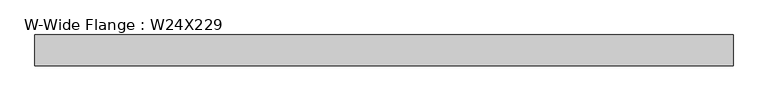
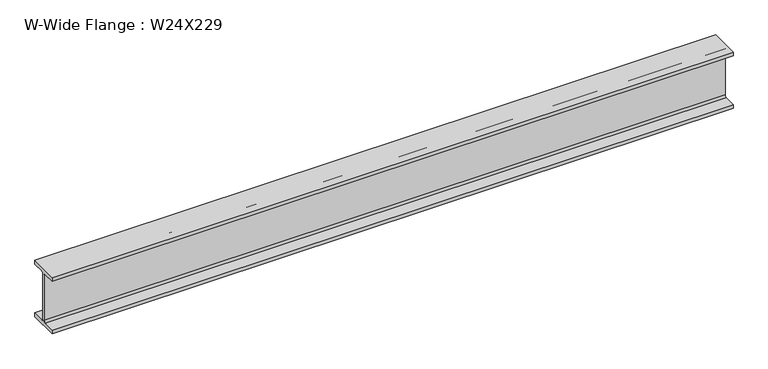
"""IFC4 building model written with IfcOpenShell, lengths in millimetres: beam geometry, W-Wide Flange : W24X229."""

from ifc_helpers import new_model, si_unit, point, frame, frame_2d, origin, place, context, project, spatial, polyline, circle_curve, trimmed, segment, composite_curve, outline, extrude, source, transform, mapped, element, save


def w_wide_flange_w24x229_eebb78a0(model_context):
    return source(origin(), model_context, "Body", "SweptSolid", [
        extrude(outline(composite_curve([segment(polyline([(-166.37, -286.258), (-34.925, -286.258)]), True, "CONTINUOUS"), segment(trimmed(circle_curve(frame_2d((-34.925, -263.525)), 22.733), [point((-34.925, -286.258))], [point((-12.192, -263.525))], True, "CARTESIAN"), True, "CONTINUOUS"), segment(polyline([(-12.192, -263.525), (-12.192, 263.525)]), True, "CONTINUOUS"), segment(trimmed(circle_curve(frame_2d((-34.925, 263.525)), 22.733), [point((-12.192, 263.525))], [point((-34.925, 286.258))], True, "CARTESIAN"), True, "CONTINUOUS"), segment(polyline([(-34.925, 286.258), (-166.37, 286.258), (-166.37, 330.2), (166.37, 330.2), (166.37, 286.258), (34.925, 286.258)]), True, "CONTINUOUS"), segment(trimmed(circle_curve(frame_2d((34.925, 263.525)), 22.733), [point((34.925, 286.258))], [point((12.192, 263.525))], True, "CARTESIAN"), True, "CONTINUOUS"), segment(polyline([(12.192, 263.525), (12.192, -263.525)]), True, "CONTINUOUS"), segment(trimmed(circle_curve(frame_2d((34.925, -263.525)), 22.733), [point((12.192, -263.525))], [point((34.925, -286.258))], True, "CARTESIAN"), True, "CONTINUOUS"), segment(polyline([(34.925, -286.258), (166.37, -286.258), (166.37, -330.2), (-166.37, -330.2), (-166.37, -286.258)]), True, "CONTINUOUS")], self_intersect=False)), frame((-3793.384977, 0.0, 0.0), z_axis=(1.0, 0.0, 0.0), x_axis=(0.0, 1.0, 0.0)), (0.0, 0.0, 1.0), 7550.785),
    ])


if __name__ == "__main__":
    model = new_model("IFC4")
    model_context = context("Model", 3, world=origin())
    ifc_project = project(units=[si_unit("LENGTHUNIT", "METRE", prefix="MILLI")], contexts=[model_context])
    site = spatial("IfcSite", under=ifc_project)
    building = spatial("IfcBuilding", under=site)
    placement = place(None, origin())
    w_wide_flange_w24x229_shape = w_wide_flange_w24x229_eebb78a0(model_context)
    element("IfcBeam", 1, ObjectType="W-Wide Flange : W24X229", at=placement, inside=building, context=model_context, shape_type="MappedRepresentation", body=[
        mapped(w_wide_flange_w24x229_shape, transform((0.0, 0.0, 0.0), x_axis=(1.0, 0.0, 0.0), y_axis=(0.0, 1.0, 0.0), z_axis=(0.0, 0.0, 1.0))),
    ])
    save(model, "model.ifc")

# Revit data of these elements
# Type "W-Wide Flange : W24X229"
#   Assembly Code = "B10"
#   W = 229
#   Start Extension Calculation [instance default] = 10' - 0"
#   Start Extension [instance default] = -0' - 0 1/2"
#   End Extension Calculation [instance default] = 10' - 0"
#   End Extension [instance default] = -0' - 0 1/2"
#   Length [instance default] = 5' - 0"
#   bf = 1' - 1.1"
#   d = 2' - 2"
#   k = 0' - 2 5/8"
#   k2 = 0' - 0.895"
#   tf = 0' - 1.73"
#   tw = 0' - 0.96"
#   A = 0.466667 SF
#   Beam Material [instance default] = Metal - Steel - ASTM A992
# Element 1 (IfcBeam, "W-Wide Flange : W24X229")
#   Materials on its faces: "Metal - Steel - ASTM A992"
# Materials
#   "Metal - Steel - ASTM A992": class "Metal", colour RGB 128 0 0, transparency 0
